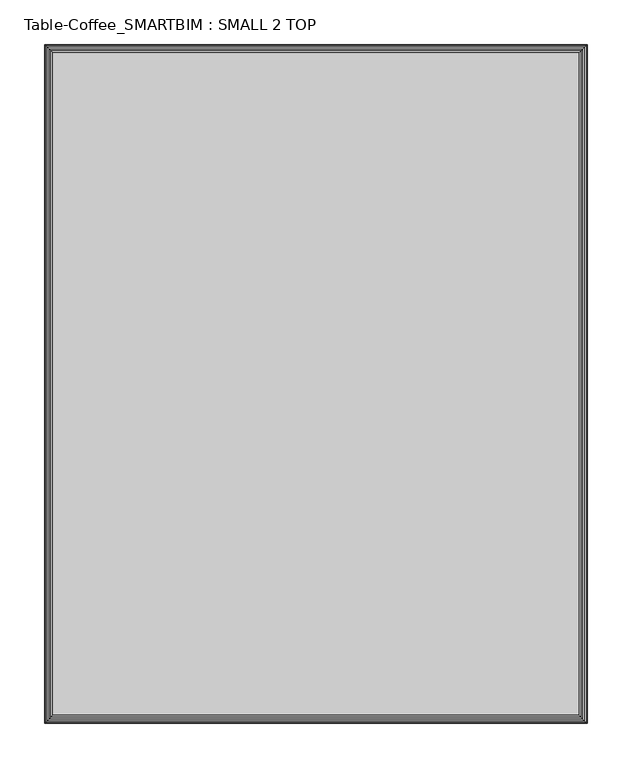
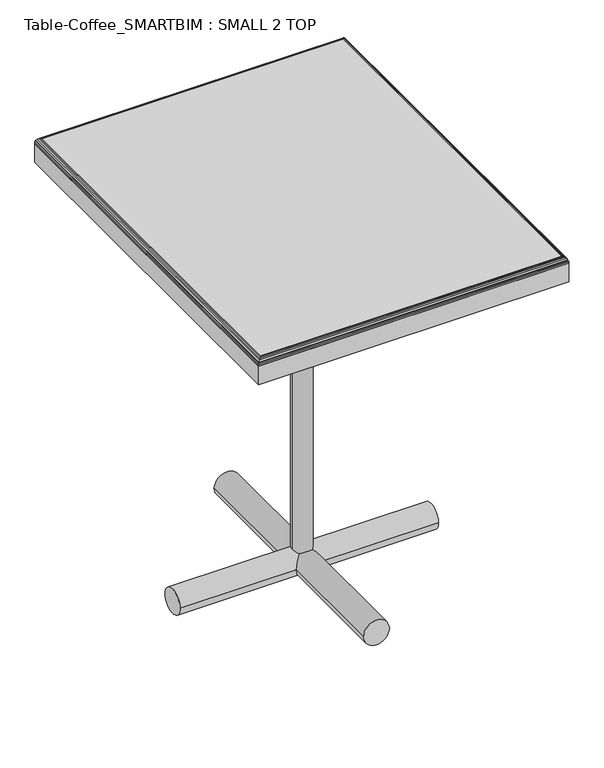
"""IFC4 building model written with IfcOpenShell, lengths in millimetres: furniture geometry, Table-Coffee_SMARTBIM : SMALL 2 TOP."""

from ifc_helpers import new_model, si_unit, point, frame, frame_2d, origin, origin_2d, place, context, project, spatial, polyline, circle_curve, ellipse_curve, trimmed, segment, composite_curve, outline, extrude, source, transform, mapped, element, save
from ifc_brep_helpers import plane_surface, cylinder_surface, advanced_brep


def table_coffee_smartbim_small_2_top_df8f75ba(model_context):
    return source(origin(), model_context, "Body", "SolidModel", [
        extrude(outline(composite_curve([segment(trimmed(circle_curve(frame_2d((0.0, 25.4)), 25.4), [point((-25.4, 25.4))], [point((25.4, 25.4))], False, "CARTESIAN"), True, "CONTINUOUS"), segment(trimmed(circle_curve(frame_2d((0.0, 25.4)), 25.4), [point((25.4, 25.4))], [point((-25.4, 25.4))], False, "CARTESIAN"), True, "CONTINUOUS")], self_intersect=False)), frame((-254.0, 0.0, 0.0), z_axis=(1.0, 0.0, 0.0), x_axis=(0.0, 1.0, 0.0)), (0.0, 0.0, 1.0), 508.0),
        extrude(outline(composite_curve([segment(trimmed(circle_curve(frame_2d((25.4, 0.0)), 25.4), [point((25.4, -25.4))], [point((25.4, 25.4))], False, "CARTESIAN"), True, "CONTINUOUS"), segment(trimmed(circle_curve(frame_2d((25.4, 0.0)), 25.4), [point((25.4, 25.4))], [point((25.4, -25.4))], False, "CARTESIAN"), True, "CONTINUOUS")], self_intersect=False)), frame((0.0, -254.0, 0.0), z_axis=(0.0, 1.0, 0.0), x_axis=(0.0, 0.0, 1.0)), (0.0, 0.0, 1.0), 508.0),
        extrude(outline(polyline([(304.8, -381.0), (-304.8, -381.0), (-304.8, 381.0), (304.8, 381.0), (304.8, -381.0)])), frame((0.0, 0.0, 723.9), z_axis=(0.0, 0.0, 1.0), x_axis=(1.0, 0.0, 0.0)), (0.0, 0.0, 1.0), 38.1),
        advanced_brep(
        [(-295.3998654, 371.5998654, 774.7), (-295.3998654, -371.5998654, 774.7), (295.3998654, -371.5998654, 774.7), (295.3998654, 371.5998654, 774.7), (304.8, -381.0, 762.0), (-304.8, -381.0, 762.0), (-304.8, 381.0, 762.0), (304.8, 381.0, 762.0), (304.8, -381.0, 765.2998654), (-304.8, -381.0, 765.2998654), (-304.8, 381.0, 765.2998654), (304.8, 381.0, 765.2998654), (-304.4372483, -380.6372483, 767.8860287), (-304.4372483, 380.6372483, 767.8860287), (-297.5616212, -373.7616212, 774.4480533), (-297.5616212, 373.7616212, 774.4480533), (-299.5639185, 375.7639185, 773.7273912), (-299.5639185, -375.7639185, 773.7273912), (-301.6885738, 377.8885738, 772.2866155), (-301.6885738, -377.8885738, 772.2866155), (-303.7102962, 379.9102962, 769.692959), (-303.7102962, -379.9102962, 769.692959), (304.4372483, 380.6372483, 767.8860287), (297.5616212, 373.7616212, 774.4480533), (299.5639185, 375.7639185, 773.7273912), (301.6885738, 377.8885738, 772.2866155), (303.7102962, 379.9102962, 769.692959), (304.4372483, -380.6372483, 767.8860287), (297.5616212, -373.7616212, 774.4480533), (299.5639185, -375.7639185, 773.7273912), (301.6885738, -377.8885738, 772.2866155), (303.7102962, -379.9102962, 769.692959)],
        [
            (0, 1),
            (1, 2),
            (2, 3),
            (3, 0),
            (4, 5),
            (5, 6),
            (6, 7),
            (7, 4),
            (4, 8),
            (8, 9),
            (9, 5),
            (9, 10),
            (10, 6),
            (10, 11),
            (11, 7),
            (11, 8),
            (9, 12, ellipse_curve(frame((-295.3998654, -371.5998654, 765.2998654), z_axis=(-0.7071067811865475, 0.7071067811865475, 0.0), x_axis=(0.7071067811865474, 0.7071067811865476, 0.0)), 13.2937978, 9.4001346)),
            (12, 13),
            (13, 10, ellipse_curve(frame((-295.3998654, 371.5998654, 765.2998654), z_axis=(-0.7071067811865475, -0.7071067811865475, 0.0), x_axis=(-0.7071067811865474, 0.7071067811865476, 0.0)), 13.2937978, 9.4001346)),
            (14, 1, ellipse_curve(frame((-295.3998654, -371.5998654, 765.2998654), z_axis=(-0.7071067811865475, 0.7071067811865475, 0.0), x_axis=(0.7071067811865474, 0.7071067811865476, 0.0)), 13.2937978, 9.4001346)),
            (0, 15, ellipse_curve(frame((-295.3998654, 371.5998654, 765.2998654), z_axis=(-0.7071067811865475, -0.7071067811865475, 0.0), x_axis=(-0.7071067811865474, 0.7071067811865476, 0.0)), 13.2937978, 9.4001346)),
            (15, 14),
            (15, 16, ellipse_curve(frame((-295.3998654, 371.5998654, 765.2998654), z_axis=(-0.7071067811865475, -0.7071067811865475, 0.0), x_axis=(-0.7071067811865474, 0.7071067811865476, 0.0)), 13.2937978, 9.4001346)),
            (16, 17),
            (17, 14, ellipse_curve(frame((-295.3998654, -371.5998654, 765.2998654), z_axis=(-0.7071067811865475, 0.7071067811865475, 0.0), x_axis=(0.7071067811865474, 0.7071067811865476, 0.0)), 13.2937978, 9.4001346)),
            (16, 18, ellipse_curve(frame((-295.3998654, 371.5998654, 765.2998654), z_axis=(-0.7071067811865475, -0.7071067811865475, 0.0), x_axis=(-0.7071067811865474, 0.7071067811865476, 0.0)), 13.2937978, 9.4001346)),
            (18, 19),
            (19, 17, ellipse_curve(frame((-295.3998654, -371.5998654, 765.2998654), z_axis=(-0.7071067811865475, 0.7071067811865475, 0.0), x_axis=(0.7071067811865474, 0.7071067811865476, 0.0)), 13.2937978, 9.4001346)),
            (18, 20, ellipse_curve(frame((-295.3998654, 371.5998654, 765.2998654), z_axis=(-0.7071067811865475, -0.7071067811865475, 0.0), x_axis=(-0.7071067811865474, 0.7071067811865476, 0.0)), 13.2937978, 9.4001346)),
            (20, 21),
            (21, 19, ellipse_curve(frame((-295.3998654, -371.5998654, 765.2998654), z_axis=(-0.7071067811865475, 0.7071067811865475, 0.0), x_axis=(0.7071067811865474, 0.7071067811865476, 0.0)), 13.2937978, 9.4001346)),
            (12, 21, ellipse_curve(frame((-295.3998654, -371.5998654, 765.2998654), z_axis=(-0.7071067811865475, 0.7071067811865475, 0.0), x_axis=(0.7071067811865474, 0.7071067811865476, 0.0)), 13.2937978, 9.4001346)),
            (20, 13, ellipse_curve(frame((-295.3998654, 371.5998654, 765.2998654), z_axis=(-0.7071067811865475, -0.7071067811865475, 0.0), x_axis=(-0.7071067811865474, 0.7071067811865476, 0.0)), 13.2937978, 9.4001346)),
            (13, 22),
            (22, 11, ellipse_curve(frame((295.3998654, 371.5998654, 765.2998654), z_axis=(-0.7071067811865475, 0.7071067811865475, 0.0), x_axis=(0.7071067811865476, 0.7071067811865474, 0.0)), 13.2937978, 9.4001346)),
            (3, 23, ellipse_curve(frame((295.3998654, 371.5998654, 765.2998654), z_axis=(-0.7071067811865475, 0.7071067811865475, 0.0), x_axis=(0.7071067811865476, 0.7071067811865474, 0.0)), 13.2937978, 9.4001346)),
            (23, 15),
            (23, 24, ellipse_curve(frame((295.3998654, 371.5998654, 765.2998654), z_axis=(-0.7071067811865475, 0.7071067811865475, 0.0), x_axis=(0.7071067811865476, 0.7071067811865474, 0.0)), 13.2937978, 9.4001346)),
            (24, 16),
            (24, 25, ellipse_curve(frame((295.3998654, 371.5998654, 765.2998654), z_axis=(-0.7071067811865475, 0.7071067811865475, 0.0), x_axis=(0.7071067811865476, 0.7071067811865474, 0.0)), 13.2937978, 9.4001346)),
            (25, 18),
            (25, 26, ellipse_curve(frame((295.3998654, 371.5998654, 765.2998654), z_axis=(-0.7071067811865475, 0.7071067811865475, 0.0), x_axis=(0.7071067811865476, 0.7071067811865474, 0.0)), 13.2937978, 9.4001346)),
            (26, 20),
            (26, 22, ellipse_curve(frame((295.3998654, 371.5998654, 765.2998654), z_axis=(-0.7071067811865475, 0.7071067811865475, 0.0), x_axis=(0.7071067811865476, 0.7071067811865474, 0.0)), 13.2937978, 9.4001346)),
            (22, 27),
            (27, 8, ellipse_curve(frame((295.3998654, -371.5998654, 765.2998654), z_axis=(0.7071067811865475, 0.7071067811865475, 0.0), x_axis=(0.7071067811865474, -0.7071067811865476, 0.0)), 13.2937978, 9.4001346)),
            (2, 28, ellipse_curve(frame((295.3998654, -371.5998654, 765.2998654), z_axis=(0.7071067811865475, 0.7071067811865475, 0.0), x_axis=(0.7071067811865474, -0.7071067811865476, 0.0)), 13.2937978, 9.4001346)),
            (28, 23),
            (28, 29, ellipse_curve(frame((295.3998654, -371.5998654, 765.2998654), z_axis=(0.7071067811865475, 0.7071067811865475, 0.0), x_axis=(0.7071067811865474, -0.7071067811865476, 0.0)), 13.2937978, 9.4001346)),
            (29, 24),
            (29, 30, ellipse_curve(frame((295.3998654, -371.5998654, 765.2998654), z_axis=(0.7071067811865475, 0.7071067811865475, 0.0), x_axis=(0.7071067811865474, -0.7071067811865476, 0.0)), 13.2937978, 9.4001346)),
            (30, 25),
            (30, 31, ellipse_curve(frame((295.3998654, -371.5998654, 765.2998654), z_axis=(0.7071067811865475, 0.7071067811865475, 0.0), x_axis=(0.7071067811865474, -0.7071067811865476, 0.0)), 13.2937978, 9.4001346)),
            (31, 26),
            (31, 27, ellipse_curve(frame((295.3998654, -371.5998654, 765.2998654), z_axis=(0.7071067811865475, 0.7071067811865475, 0.0), x_axis=(0.7071067811865474, -0.7071067811865476, 0.0)), 13.2937978, 9.4001346)),
            (27, 12),
            (14, 28),
            (17, 29),
            (19, 30),
            (21, 31),
        ],
        [
            plane_surface(frame((-304.8, -381.0, 774.7), z_axis=(0.0, 0.0, 1.0), x_axis=(-1.0, 0.0, 0.0))),
            plane_surface(frame((-304.8, -381.0, 762.0), z_axis=(0.0, 0.0, -1.0), x_axis=(1.0, 0.0, 0.0))),
            plane_surface(frame((304.8, -381.0, 774.7), z_axis=(0.0, -1.0, 0.0), x_axis=(0.0, 0.0, -1.0))),
            plane_surface(frame((-304.8, -381.0, 774.7), z_axis=(-1.0, 0.0, 0.0), x_axis=(0.0, 0.0, -1.0))),
            plane_surface(frame((-304.8, 381.0, 774.7), z_axis=(0.0, 1.0, 0.0), x_axis=(0.0, 0.0, -1.0))),
            plane_surface(frame((304.8, 381.0, 774.7), z_axis=(1.0, 0.0, 0.0), x_axis=(0.0, 0.0, -1.0))),
            cylinder_surface(frame((-295.3998654, -381.0, 765.2998654), z_axis=(0.0, 1.0, 0.0), x_axis=(1.0, 0.0, 0.0)), 9.4001346),
            cylinder_surface(frame((-304.8, 371.5998654, 765.2998654), z_axis=(1.0, 0.0, 0.0), x_axis=(0.0, -1.0, 0.0)), 9.4001346),
            cylinder_surface(frame((295.3998654, 381.0, 765.2998654), z_axis=(0.0, -1.0, 0.0), x_axis=(-1.0, 0.0, 0.0)), 9.4001346),
            cylinder_surface(frame((304.8, -371.5998654, 765.2998654), z_axis=(-1.0, 0.0, 0.0), x_axis=(0.0, 1.0, 0.0)), 9.4001346),
        ],
        [
            (0, [[1, 2, 3, 4]]),
            (1, [[5, 6, 7, 8]]),
            (2, [[9, 10, 11, -5]]),
            (3, [[-11, 12, 13, -6]]),
            (4, [[-13, 14, 15, -7]]),
            (5, [[-15, 16, -9, -8]]),
            (6, [[-12, 17, 18, 19]]),
            (6, [[20, -1, 21, 22]]),
            (6, [[23, 24, 25, -22]]),
            (6, [[26, 27, 28, -24]]),
            (6, [[29, 30, 31, -27]]),
            (6, [[32, -30, 33, -18]]),
            (7, [[34, 35, -14, -19]]),
            (7, [[-4, 36, 37, -21]]),
            (7, [[-37, 38, 39, -23]]),
            (7, [[-39, 40, 41, -26]]),
            (7, [[-41, 42, 43, -29]]),
            (7, [[-43, 44, -34, -33]]),
            (8, [[45, 46, -16, -35]]),
            (8, [[-3, 47, 48, -36]]),
            (8, [[-48, 49, 50, -38]]),
            (8, [[-50, 51, 52, -40]]),
            (8, [[-52, 53, 54, -42]]),
            (8, [[-54, 55, -45, -44]]),
            (9, [[-10, -46, 56, -17]]),
            (9, [[57, -47, -2, -20]]),
            (9, [[58, -49, -57, -25]]),
            (9, [[59, -51, -58, -28]]),
            (9, [[60, -53, -59, -31]]),
            (9, [[-56, -55, -60, -32]]),
        ],
    ),
        extrude(outline(polyline([(76.2, -76.2), (-76.2, -76.2), (-76.2, 76.2), (76.2, 76.2), (76.2, -76.2)])), frame((0.0, 0.0, 755.65), z_axis=(0.0, 0.0, 1.0), x_axis=(1.0, 0.0, 0.0)), (0.0, 0.0, 1.0), 6.35),
        extrude(outline(composite_curve([segment(trimmed(circle_curve(origin_2d(), 19.05), [point((-19.05, 0.0))], [point((19.05, 0.0))], False, "CARTESIAN"), True, "CONTINUOUS"), segment(trimmed(circle_curve(origin_2d(), 19.05), [point((19.05, 0.0))], [point((-19.05, 0.0))], False, "CARTESIAN"), True, "CONTINUOUS")], self_intersect=False)), frame((0.0, 0.0, 24.2070278), z_axis=(0.0, 0.0, 1.0), x_axis=(1.0, 0.0, 0.0)), (0.0, 0.0, 1.0), 731.4429722),
    ])


if __name__ == "__main__":
    model = new_model("IFC4")
    model_context = context("Model", 3, world=origin())
    ifc_project = project(units=[si_unit("LENGTHUNIT", "METRE", prefix="MILLI")], contexts=[model_context])
    site = spatial("IfcSite", under=ifc_project)
    building = spatial("IfcBuilding", under=site)
    placement = place(None, origin())
    table_coffee_smartbim_small_2_top_shape = table_coffee_smartbim_small_2_top_df8f75ba(model_context)
    element("IfcFurniture", 1, ObjectType="Table-Coffee_SMARTBIM : SMALL 2 TOP", at=placement, inside=building, context=model_context, shape_type="MappedRepresentation", body=[
        mapped(table_coffee_smartbim_small_2_top_shape, transform((0.0, 0.0, 0.0), x_axis=(1.0, 0.0, 0.0), y_axis=(0.0, 1.0, 0.0), z_axis=(0.0, 0.0, 1.0))),
    ])
    save(model, "model.ifc")

# Revit data of these elements
# Type "Table-Coffee_SMARTBIM : SMALL 2 TOP"
#   Subcategory = "Table\r\n"
#   SmartBIM Object Created By = "SMARTBIM, LLC"
#   Manufacturer = "SMARTBIM"
#   Assembly Code = "E2020200"
#   95 CSI = "12500"
#   04 CSI = "12 50 00"
#   table cloth = 0' - 1 1/2"
#   Width = 2' - 0"
#   SmartBIM Object Version = 3
#   Height = 2' - 6"
#   Depth = 2' - 6"
#   Default Elevation = 4' - 0"
#   white cloth_parameter = Sals Wood
#   Table Unit = MET
#   Glide = none
#   Glass = none
# Element 1 (IfcFurniture, "Table-Coffee_SMARTBIM : SMALL 2 TOP")
#   Materials on its faces: "Sals Wood", "MET"
# Materials
#   "Sals Wood": class "Wood", colour RGB 198 202 183, transparency 0, Description = "Generic wood", Cost = 0
#   "MET": class "Metal", colour RGB 189 187 185, transparency 0
